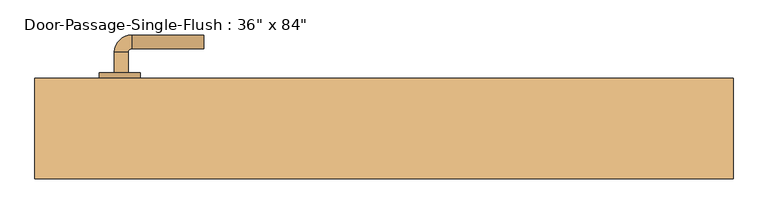
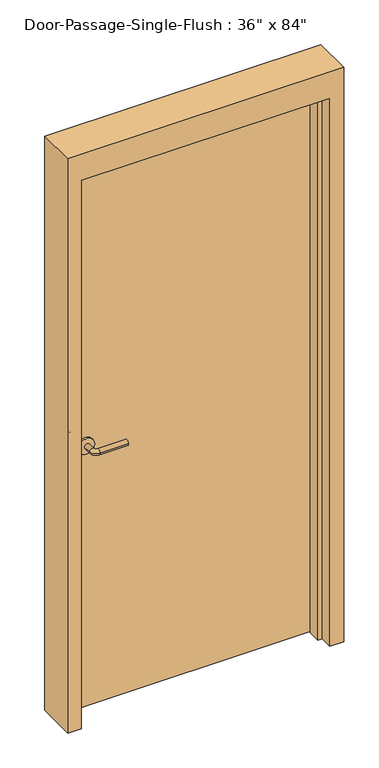
"""IFC4 building model written with IfcOpenShell, lengths in millimetres: door geometry."""

from ifc_helpers import new_model, si_unit, point, frame, frame_2d, origin, origin_with_axes, place, context, project, spatial, polyline, circle_curve, ellipse_curve, trimmed, segment, composite_curve, outline, extrude, faceted_brep, source, transform, mapped, element, save
from ifc_brep_helpers import plane_surface, cylinder_surface, revolved_surface, advanced_brep


def door_a8315dbd(model_context):
    return source(origin(), model_context, "Body", "SolidModel", [
        advanced_brep(
        [(-392.190625, 15.8125, 1016.0), (-372.190625, 15.8125, 1016.0), (-372.190625, -14.1875, 1016.0), (-392.190625, -14.1875, 1016.0), (-367.190625, -19.1875, 1016.0), (-367.190625, -39.1875, 1016.0), (-262.190625, -39.1875, 1016.0), (-262.190625, -19.1875, 1016.0)],
        [
            (0, 1, circle_curve(frame((-382.190625, 15.8125, 1016.0), z_axis=(0.0, 1.0, 0.0), x_axis=(1.0, 0.0, 0.0)), 10.0)),
            (1, 0, circle_curve(frame((-382.190625, 15.8125, 1016.0), z_axis=(0.0, 1.0, 0.0), x_axis=(1.0, 0.0, 0.0)), 10.0)),
            (1, 2),
            (2, 3, circle_curve(frame((-382.190625, -14.1875, 1016.0), z_axis=(0.0, 1.0, 0.0), x_axis=(1.0, 0.0, 0.0)), 10.0)),
            (3, 0),
            (3, 2, circle_curve(frame((-382.190625, -14.1875, 1016.0), z_axis=(0.0, 1.0, 0.0), x_axis=(1.0, 0.0, 0.0)), 10.0)),
            (4, 5, circle_curve(frame((-367.190625, -29.1875, 1016.0), z_axis=(-1.0, 0.0, 0.0), x_axis=(0.0, 1.0, 0.0)), 10.0)),
            (5, 3, circle_curve(frame((-367.190625, -14.1875, 1016.0), z_axis=(0.0, 0.0, -1.0), x_axis=(-1.0, 0.0, 0.0)), 25.0)),
            (2, 4, circle_curve(frame((-367.190625, -14.1875, 1016.0), z_axis=(0.0, 0.0, 1.0), x_axis=(-1.0, 0.0, 0.0)), 5.0)),
            (5, 4, circle_curve(frame((-367.190625, -29.1875, 1016.0), z_axis=(-1.0, 0.0, 0.0), x_axis=(0.0, 1.0, 0.0)), 10.0)),
            (6, 7, circle_curve(frame((-262.190625, -29.1875, 1016.0), z_axis=(1.0, 0.0, 0.0), x_axis=(0.0, 1.0, 0.0)), 10.0)),
            (7, 6, circle_curve(frame((-262.190625, -29.1875, 1016.0), z_axis=(1.0, 0.0, 0.0), x_axis=(0.0, 1.0, 0.0)), 10.0)),
            (4, 7),
            (6, 5),
        ],
        [
            plane_surface(frame((-382.190625, 15.8125, 1016.0), z_axis=(0.0, 1.0, 0.0), x_axis=(0.0, 0.0, 1.0))),
            cylinder_surface(frame((-382.190625, 15.8125, 1016.0), z_axis=(0.0, 1.0, 0.0), x_axis=(1.0, 0.0, 0.0)), 10.0),
            revolved_surface(trimmed(ellipse_curve(frame((-382.190625, -14.1875, 1016.0), z_axis=(0.0, -1.0, 0.0), x_axis=(1.0, 0.0, 0.0)), 10.0, 10.0), [point((-392.190625, -14.1875, 1016.0))], [point((-372.190625, -14.1875, 1016.0))], True, "CARTESIAN"), (-367.190625, -14.1875, 1016.0), (0.0, 0.0, -1.0)),
            revolved_surface(trimmed(ellipse_curve(frame((-382.190625, -14.1875, 1016.0), z_axis=(0.0, -1.0, 0.0), x_axis=(1.0, 0.0, 0.0)), 10.0, 10.0), [point((-372.190625, -14.1875, 1016.0))], [point((-392.190625, -14.1875, 1016.0))], True, "CARTESIAN"), (-367.190625, -14.1875, 1016.0), (0.0, 0.0, -1.0)),
            plane_surface(frame((-262.190625, -29.1875, 1016.0), z_axis=(1.0, 0.0, 0.0), x_axis=(0.0, 0.0, 1.0))),
            cylinder_surface(frame((-367.190625, -29.1875, 1016.0), z_axis=(-1.0, 0.0, 0.0), x_axis=(0.0, 1.0, 0.0)), 10.0),
        ],
        [
            (0, [[1, 2]]),
            (1, [[3, 4, 5, -2]]),
            (1, [[-5, 6, -3, -1]]),
            (2, [[7, 8, -4, 9]]),
            (3, [[10, -9, -6, -8]]),
            (4, [[11, 12]]),
            (5, [[13, -11, 14, -7]]),
            (5, [[-14, -12, -13, -10]]),
        ],
    ),
        extrude(outline(composite_curve([segment(trimmed(circle_curve(frame_2d((1016.0, -384.690625)), 30.0), [point((1016.0, -414.690625))], [point((1016.0, -354.690625))], False, "CARTESIAN"), True, "CONTINUOUS"), segment(trimmed(circle_curve(frame_2d((1016.0, -384.690625)), 30.0), [point((1016.0, -354.690625))], [point((1016.0, -414.690625))], False, "CARTESIAN"), True, "CONTINUOUS")], self_intersect=False)), frame((0.0, 15.8125, 0.0), z_axis=(0.0, 1.0, 0.0), x_axis=(0.0, 0.0, 1.0)), (0.0, 0.0, 1.0), 8.0),
        advanced_brep(
        [(-392.190625, 76.2625, 1016.0), (-372.190625, 76.2625, 1016.0), (-392.190625, 106.2625, 1016.0), (-372.190625, 106.2625, 1016.0), (-367.190625, 111.2625, 1016.0), (-367.190625, 131.2625, 1016.0), (-262.190625, 131.2625, 1016.0), (-262.190625, 111.2625, 1016.0)],
        [
            (0, 1, circle_curve(frame((-382.190625, 76.2625, 1016.0), z_axis=(0.0, -1.0, 0.0), x_axis=(1.0, 0.0, 0.0)), 10.0)),
            (1, 0, circle_curve(frame((-382.190625, 76.2625, 1016.0), z_axis=(0.0, -1.0, 0.0), x_axis=(1.0, 0.0, 0.0)), 10.0)),
            (0, 2),
            (2, 3, circle_curve(frame((-382.190625, 106.2625, 1016.0), z_axis=(0.0, -1.0, 0.0), x_axis=(1.0, 0.0, 0.0)), 10.0)),
            (3, 1),
            (3, 2, circle_curve(frame((-382.190625, 106.2625, 1016.0), z_axis=(0.0, -1.0, 0.0), x_axis=(1.0, 0.0, 0.0)), 10.0)),
            (4, 3, circle_curve(frame((-367.190625, 106.2625, 1016.0), z_axis=(0.0, 0.0, 1.0), x_axis=(-1.0, 0.0, 0.0)), 5.0)),
            (2, 5, circle_curve(frame((-367.190625, 106.2625, 1016.0), z_axis=(0.0, 0.0, -1.0), x_axis=(-1.0, 0.0, 0.0)), 25.0)),
            (5, 4, circle_curve(frame((-367.190625, 121.2625, 1016.0), z_axis=(-1.0, 0.0, 0.0), x_axis=(0.0, -1.0, 0.0)), 10.0)),
            (4, 5, circle_curve(frame((-367.190625, 121.2625, 1016.0), z_axis=(-1.0, 0.0, 0.0), x_axis=(0.0, -1.0, 0.0)), 10.0)),
            (6, 7, circle_curve(frame((-262.190625, 121.2625, 1016.0), z_axis=(1.0, 0.0, 0.0), x_axis=(0.0, -1.0, 0.0)), 10.0)),
            (7, 6, circle_curve(frame((-262.190625, 121.2625, 1016.0), z_axis=(1.0, 0.0, 0.0), x_axis=(0.0, -1.0, 0.0)), 10.0)),
            (5, 6),
            (7, 4),
        ],
        [
            plane_surface(frame((-382.190625, 76.2625, 1016.0), z_axis=(0.0, -1.0, 0.0), x_axis=(0.0, 0.0, 1.0))),
            cylinder_surface(frame((-382.190625, 76.2625, 1016.0), z_axis=(0.0, -1.0, 0.0), x_axis=(1.0, 0.0, 0.0)), 10.0),
            revolved_surface(trimmed(ellipse_curve(frame((-382.190625, 106.2625, 1016.0), z_axis=(0.0, -1.0, 0.0), x_axis=(1.0, 0.0, 0.0)), 10.0, 10.0), [point((-392.190625, 106.2625, 1016.0))], [point((-372.190625, 106.2625, 1016.0))], True, "CARTESIAN"), (-367.190625, 106.2625, 1016.0), (0.0, 0.0, -1.0)),
            revolved_surface(trimmed(ellipse_curve(frame((-382.190625, 106.2625, 1016.0), z_axis=(0.0, -1.0, 0.0), x_axis=(1.0, 0.0, 0.0)), 10.0, 10.0), [point((-372.190625, 106.2625, 1016.0))], [point((-392.190625, 106.2625, 1016.0))], True, "CARTESIAN"), (-367.190625, 106.2625, 1016.0), (0.0, 0.0, -1.0)),
            plane_surface(frame((-262.190625, 121.2625, 1016.0), z_axis=(1.0, 0.0, 0.0), x_axis=(0.0, 0.0, 1.0))),
            cylinder_surface(frame((-367.190625, 121.2625, 1016.0), z_axis=(-1.0, 0.0, 0.0), x_axis=(0.0, -1.0, 0.0)), 10.0),
        ],
        [
            (0, [[1, 2]]),
            (1, [[-1, 3, 4, 5]]),
            (1, [[-2, -5, 6, -3]]),
            (2, [[7, -4, 8, 9]]),
            (3, [[-8, -6, -7, 10]]),
            (4, [[11, 12]]),
            (5, [[-9, 13, -12, 14]]),
            (5, [[-10, -14, -11, -13]]),
        ],
    ),
        extrude(outline(composite_curve([segment(trimmed(circle_curve(frame_2d((1016.0, -384.690625)), 30.0), [point((1016.0, -414.690625))], [point((1016.0, -354.690625))], False, "CARTESIAN"), True, "CONTINUOUS"), segment(trimmed(circle_curve(frame_2d((1016.0, -384.690625)), 30.0), [point((1016.0, -354.690625))], [point((1016.0, -414.690625))], False, "CARTESIAN"), True, "CONTINUOUS")], self_intersect=False)), frame((0.0, 68.2625, 0.0), z_axis=(0.0, 1.0, 0.0), x_axis=(0.0, 0.0, 1.0)), (0.0, 0.0, 1.0), 8.0),
        faceted_brep([(457.2, 19.05, 0.0), (457.2, 68.2625, 0.0), (508.0, 68.2625, 0.0), (508.0, -77.7875, 0.0), (457.2, -77.7875, 0.0), (457.2, -28.575, 0.0), (441.325, -28.575, 0.0), (441.325, 19.05, 0.0), (457.2, 19.05, 2133.6), (457.2, 68.2625, 2133.6), (-457.2, 68.2625, 2133.6), (-457.2, 68.2625, 0.0), (-508.0, 68.2625, 0.0), (-508.0, 68.2625, 2235.2), (508.0, 68.2625, 2235.2), (508.0, -77.7875, 2235.2), (-508.0, -77.7875, 2235.2), (-508.0, -77.7875, 0.0), (-457.2, -77.7875, 0.0), (-457.2, -77.7875, 2133.6), (457.2, -77.7875, 2133.6), (457.2, -28.575, 2133.6), (-457.2, -28.575, 2133.6), (-457.2, -28.575, 0.0), (-441.325, -28.575, 0.0), (-441.325, -28.575, 2117.725), (441.325, -28.575, 2117.725), (441.325, 19.05, 2117.725), (-441.325, 19.05, 2117.725), (-441.325, 19.05, 0.0), (-457.2, 19.05, 0.0), (-457.2, 19.05, 2133.6)], [[[0, 1, 2, 3, 4, 5, 6, 7]], [[1, 0, 8, 9]], [[2, 1, 9, 10, 11, 12, 13, 14]], [[3, 2, 14, 15]], [[4, 3, 15, 16, 17, 18, 19, 20]], [[5, 4, 20, 21]], [[6, 5, 21, 22, 23, 24, 25, 26]], [[7, 6, 26, 27]], [[0, 7, 27, 28, 29, 30, 31, 8]], [[9, 8, 31, 10]], [[20, 19, 22, 21]], [[26, 25, 28, 27]], [[12, 11, 30, 29, 24, 23, 18, 17]], [[11, 10, 31, 30]], [[13, 12, 17, 16]], [[19, 18, 23, 22]], [[25, 24, 29, 28]], [[15, 14, 13, 16]]]),
        extrude(outline(polyline([(457.2, 23.8125), (-457.2, 23.8125), (-457.2, 68.2625), (457.2, 68.2625), (457.2, 23.8125)])), origin_with_axes(), (0.0, 0.0, 1.0), 2133.6),
    ])


if __name__ == "__main__":
    model = new_model("IFC4")
    model_context = context("Model", 3, world=origin())
    ifc_project = project(units=[si_unit("LENGTHUNIT", "METRE", prefix="MILLI")], contexts=[model_context])
    site = spatial("IfcSite", under=ifc_project)
    building = spatial("IfcBuilding", under=site)
    placement = place(None, origin())
    door_shape = door_a8315dbd(model_context)
    element("IfcDoor", 1, ObjectType="Door-Passage-Single-Flush : 36\" x 84\"", at=placement, inside=building, context=model_context, shape_type="MappedRepresentation", body=[
        mapped(door_shape, transform((0.0, 0.0, 0.0), x_axis=(1.0, 0.0, 0.0), y_axis=(0.0, 1.0, 0.0), z_axis=(0.0, 0.0, 1.0))),
    ])
    save(model, "model.ifc")

# Revit data of these elements
# Type "Door-Passage-Single-Flush : 36\" x 84\""
#   Type Mark = "35"
#   Assembly Code = "B2030200"
#   Analytic Construction = "Wooden"
#   Thickness = 0' - 1 3/4"
#   Thermal Resistance (R) = 2.5876 (h·ft²·°F)/BTU
#   Swing Angle [instance default] = 90.00°
#   Strike Height = 3' - 4"
#   Rough Width [instance default] = 3' - 4"
#   Rough Height [instance default] = 7' - 4"
#   MF Opening Height [instance default] = 0' - 4"
#   MF Opening Width [instance default] = 0' - 4"
#   Inset Calculate [instance default] = 0' - 4"
#   Masonry Inset [instance default] = 0' - 1"
#   Height = 7' - 0"
#   Width = 3' - 0"
#   Heat Transfer Coefficient (U) = 0.3865 BTU/(h·ft²·°F)
#   Masonry Frame Depth = 0' - 5 3/4"
#   Masonry Frame [instance default] = yes
#   Function = 1
#   Dry Wall Frame [instance default] = no
#   Panel Material = Wood - Birch
#   Frame Material = Metal - Paint Finish - Grey
#   Door Handle Material = Aluminum
#   Visual Light Transmittance = 0
#   Solar Heat Gain Coefficient = 0
#   Wall Closure = (empty or 0)
# Element 1 (IfcDoor, "Door-Passage-Single-Flush : 36\" x 84\"")
#   Inset Calculate = 0' - 3"
#   Masonry Inset = 0' - 0"
#   Materials on its faces: "Aluminum", "Metal - Paint Finish - Grey", "Wood - Birch"
# Materials
#   "Wood - Birch": class "Wood", colour RGB 166 116 52, transparency 0, Cost = 0
#   "Metal - Paint Finish - Grey": class "Paint", colour RGB 104 104 104, transparency 0, Cost = 0
#   "Aluminum": class "Metal", colour RGB 247 247 247, transparency 0, Description = "Aluminum 6061", Cost = 0
